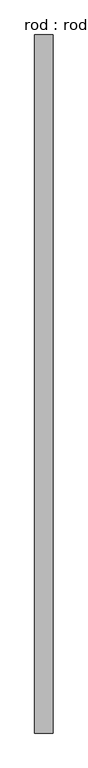
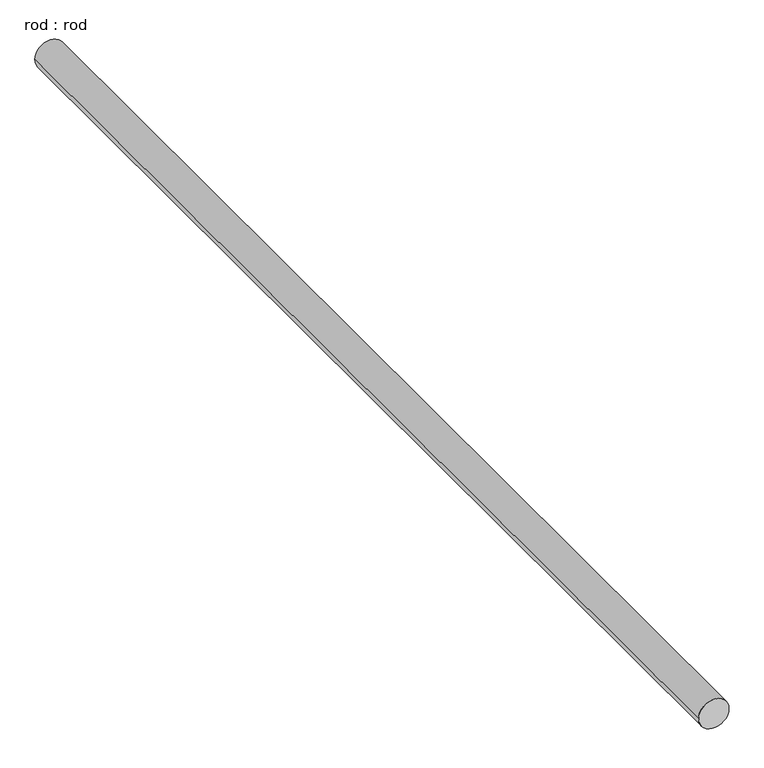
"""IFC4 building model written with IfcOpenShell, lengths in millimetres: proxy geometry, rod : rod."""

from ifc_helpers import new_model, si_unit, point, frame, frame_2d, origin, place, context, project, spatial, circle_curve, trimmed, segment, composite_curve, outline, extrude, source, transform, mapped, element, save


def rod_rod_934cf544(model_context):
    return source(origin(), model_context, "Body", "SweptSolid", [
        extrude(outline(composite_curve([segment(trimmed(circle_curve(frame_2d((0.0108462, 0.0)), 200.0), [point((0.0108462, 200.0))], [point((0.0108462, -200.0))], False, "CARTESIAN"), True, "CONTINUOUS"), segment(trimmed(circle_curve(frame_2d((0.0108462, 0.0)), 200.0), [point((0.0108462, -200.0))], [point((0.0108462, 200.0))], False, "CARTESIAN"), True, "CONTINUOUS")], self_intersect=False)), frame((0.0, -3460.8428132, 0.0), z_axis=(0.0, 1.0, 0.0), x_axis=(0.0, 0.0, 1.0)), (0.0, 0.0, 1.0), 15107.1428571),
    ])


if __name__ == "__main__":
    model = new_model("IFC4")
    model_context = context("Model", 3, world=origin())
    ifc_project = project(units=[si_unit("LENGTHUNIT", "METRE", prefix="MILLI")], contexts=[model_context])
    site = spatial("IfcSite", under=ifc_project)
    building = spatial("IfcBuilding", under=site)
    placement = place(None, origin())
    rod_rod_shape = rod_rod_934cf544(model_context)
    element("IfcBuildingElementProxy", 1, Name="rod : rod", ObjectType="rod : rod", at=placement, inside=building, context=model_context, shape_type="MappedRepresentation", body=[
        mapped(rod_rod_shape, transform((0.0, 0.0, 0.0), x_axis=(1.0, 0.0, 0.0), y_axis=(0.0, 1.0, 0.0), z_axis=(0.0, 0.0, 1.0))),
    ])
    save(model, "model.ifc")

# Revit data of these elements
# Type "rod : rod"
#   Default Elevation = 0
